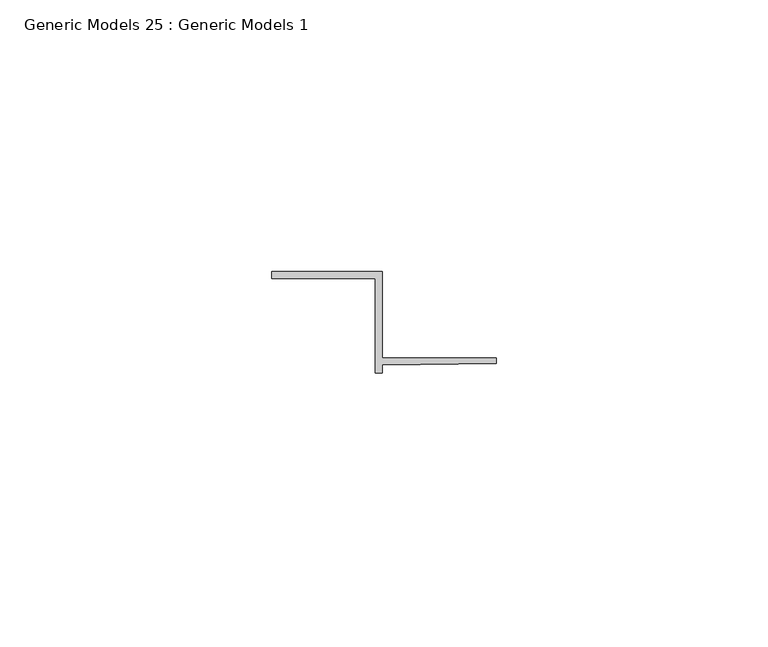
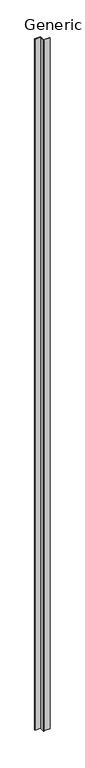
"""IFC4 building model written with IfcOpenShell, lengths in millimetres: proxy geometry, Generic Models 25 : Generic Models 1."""

from ifc_helpers import new_model, si_unit, frame, origin, place, context, project, spatial, polyline, outline, extrude, source, transform, mapped, element, save


def generic_models_25_generic_models_1_c4aab125(model_context):
    return source(origin(), model_context, "Body", "SweptSolid", [
        extrude(outline(polyline([(14867.5042846, 5573.2717424), (14866.2342846, 5573.2717424), (14866.2342846, 5590.6707424), (14847.1842846, 5590.6707424), (14847.1842846, 5591.9407424), (14867.5042846, 5591.9407424), (14867.5042846, 5576.0657424), (14888.4592748, 5576.0657424), (14888.4592748, 5575.0560127), (14867.5042846, 5574.7957424), (14867.5042846, 5573.2717424)])), frame((0.0, 0.0, 450.7860265), z_axis=(0.0, 0.0, 1.0), x_axis=(1.0, 0.0, 0.0)), (0.0, 0.0, 1.0), 2444.75),
    ])


if __name__ == "__main__":
    model = new_model("IFC4")
    model_context = context("Model", 3, world=origin())
    ifc_project = project(units=[si_unit("LENGTHUNIT", "METRE", prefix="MILLI")], contexts=[model_context])
    site = spatial("IfcSite", under=ifc_project)
    building = spatial("IfcBuilding", under=site)
    placement = place(None, origin())
    generic_models_25_generic_models_1_shape = generic_models_25_generic_models_1_c4aab125(model_context)
    element("IfcBuildingElementProxy", 1, Name="Generic Models 25 : Generic Models 1", ObjectType="Generic Models 25 : Generic Models 1", at=placement, inside=building, context=model_context, shape_type="MappedRepresentation", body=[
        mapped(generic_models_25_generic_models_1_shape, transform((0.0, 0.0, 0.0), x_axis=(1.0, 0.0, 0.0), y_axis=(0.0, 1.0, 0.0), z_axis=(0.0, 0.0, 1.0))),
    ])
    save(model, "model.ifc")

# Revit data of these elements
# Element 1 (IfcBuildingElementProxy, "Generic Models 25 : Generic Models 1")
#   Materials on its faces: "ALUM. FRY REGLET - Z REVEAL"
# Materials
#   "ALUM. FRY REGLET - Z REVEAL": class "Unassigned", colour RGB 226 225 224, transparency 0, Cost = 0
